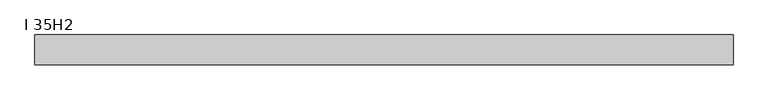
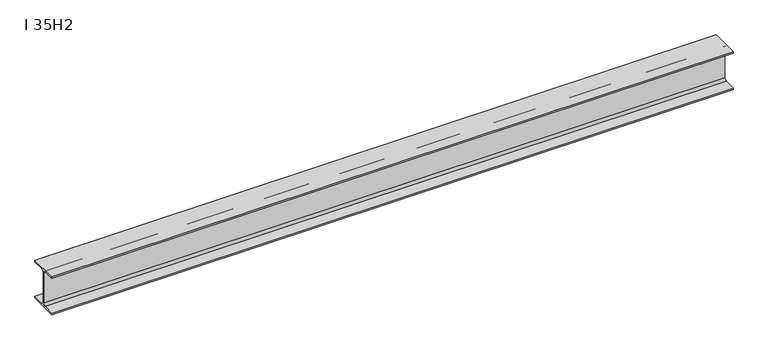
"""IFC4 building model written with IfcOpenShell, lengths in millimetres: beam geometry, Двутавр широкополочный (ГОСТ 26020-83) : I 35H2."""

from ifc_helpers import new_model, si_unit, point, frame, frame_2d, origin, place, context, project, spatial, polyline, circle_curve, trimmed, segment, composite_curve, outline, extrude, source, transform, mapped, element, save


def i_35h2_85f5d5b2(model_context):
    return source(origin(), model_context, "Body", "SweptSolid", [
        extrude(outline(composite_curve([segment(polyline([(125.0, -156.5), (125.0, -170.5), (-125.0, -170.5), (-125.0, -156.5), (-25.0, -156.5)]), True, "CONTINUOUS"), segment(trimmed(circle_curve(frame_2d((-25.0, -136.5)), 20.0), [point((-25.0, -156.5))], [point((-5.0, -136.5))], True, "CARTESIAN"), True, "CONTINUOUS"), segment(polyline([(-5.0, -136.5), (-5.0, 136.5)]), True, "CONTINUOUS"), segment(trimmed(circle_curve(frame_2d((-25.0, 136.5)), 20.0), [point((-5.0, 136.5))], [point((-25.0, 156.5))], True, "CARTESIAN"), True, "CONTINUOUS"), segment(polyline([(-25.0, 156.5), (-125.0, 156.5), (-125.0, 170.5), (125.0, 170.5), (125.0, 156.5), (25.0, 156.5)]), True, "CONTINUOUS"), segment(trimmed(circle_curve(frame_2d((25.0, 136.5)), 20.0), [point((25.0, 156.5))], [point((5.0, 136.5))], True, "CARTESIAN"), True, "CONTINUOUS"), segment(polyline([(5.0, 136.5), (5.0, -136.5)]), True, "CONTINUOUS"), segment(trimmed(circle_curve(frame_2d((25.0, -136.5)), 20.0), [point((5.0, -136.5))], [point((25.0, -156.5))], True, "CARTESIAN"), True, "CONTINUOUS"), segment(polyline([(25.0, -156.5), (125.0, -156.5)]), True, "CONTINUOUS")], self_intersect=False)), frame((-2904.0, 0.0, 0.0), z_axis=(1.0, 0.0, 0.0), x_axis=(0.0, 1.0, 0.0)), (0.0, 0.0, 1.0), 5808.0),
    ])


if __name__ == "__main__":
    model = new_model("IFC4")
    model_context = context("Model", 3, world=origin())
    ifc_project = project(units=[si_unit("LENGTHUNIT", "METRE", prefix="MILLI")], contexts=[model_context])
    site = spatial("IfcSite", under=ifc_project)
    building = spatial("IfcBuilding", under=site)
    placement = place(None, origin())
    i_35h2_shape = i_35h2_85f5d5b2(model_context)
    element("IfcBeam", 1, ObjectType="Двутавр широкополочный (ГОСТ 26020-83) : I 35H2", at=placement, inside=building, context=model_context, shape_type="MappedRepresentation", body=[
        mapped(i_35h2_shape, transform((0.0, 0.0, 0.0), x_axis=(1.0, 0.0, 0.0), y_axis=(0.0, 1.0, 0.0), z_axis=(0.0, 0.0, 1.0))),
    ])
    save(model, "model.ifc")

# Revit data of these elements
# Type "Двутавр широкополочный (ГОСТ 26020-83) : I 35H2"
#   ra = 20 mm
#   W = 0.806107
#   Vz = 170.5 mm
#   Vy = 125 mm
#   Vpz = 170.5 mm
#   Vpy = 125 mm
#   Length [instance default] = 1500 mm
#   bf = 250 mm
#   d = 341 mm
#   tf = 14 mm
#   tw = 10 mm
#   A = 0.010474 m²
#   Structural Material [instance default] = Металл - Сталь - 345 МПa
#   Assembly Code = ""
# Element 1 (IfcBeam, "Двутавр широкополочный (ГОСТ 26020-83) : I 35H2")
#   Structural Material = C235
#   Materials on its faces: "C235"
# Materials
#   "Металл - Сталь - 345 МПa": class "Металл", colour RGB 247 247 247, transparency 0
#   "C235": class "Не назначено", colour RGB 0 0 0, transparency 0
